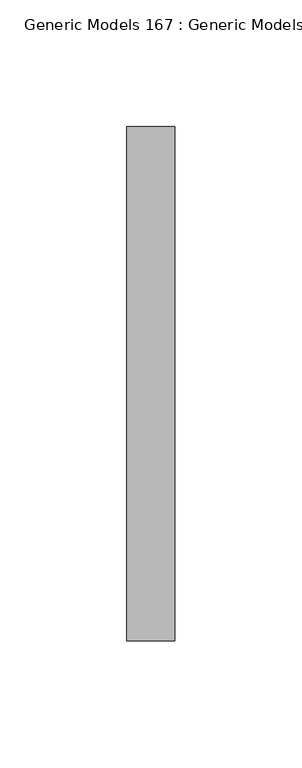
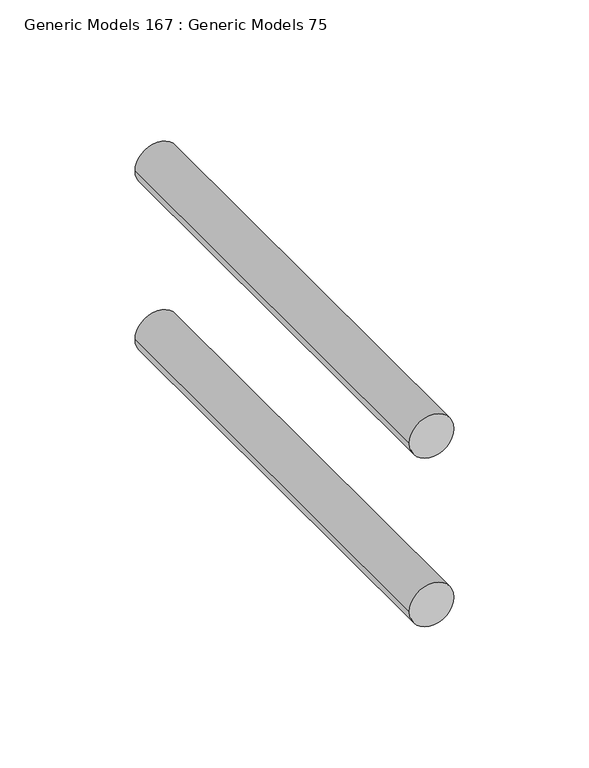
"""IFC4 building model written with IfcOpenShell, lengths in millimetres: proxy geometry, Generic Models 167 : Generic Models 75."""

from ifc_helpers import new_model, si_unit, point, frame, frame_2d, origin, place, context, project, spatial, circle_curve, trimmed, segment, composite_curve, outline, extrude, source, transform, mapped, element, save


def generic_models_167_generic_models_75_c1ef55c6(model_context):
    return source(origin(), model_context, "Body", "SweptSolid", [
        extrude(outline(composite_curve([segment(trimmed(circle_curve(frame_2d((271765.7125, 31975.4096032)), 9.525), [point((271765.7125, 31965.8846032))], [point((271765.7125, 31984.9346032))], False, "CARTESIAN"), True, "CONTINUOUS"), segment(trimmed(circle_curve(frame_2d((271765.7125, 31975.4096032)), 9.525), [point((271765.7125, 31984.9346032))], [point((271765.7125, 31965.8846032))], False, "CARTESIAN"), True, "CONTINUOUS")], self_intersect=False)), frame((0.0, 30672.7406612, 0.0), z_axis=(0.0, 1.0, 0.0), x_axis=(0.0, 0.0, 1.0)), (0.0, 0.0, 1.0), 203.2),
        extrude(outline(composite_curve([segment(trimmed(circle_curve(frame_2d((271841.9125, 31975.4096032)), 9.525), [point((271841.9125, 31965.8846032))], [point((271841.9125, 31984.9346032))], False, "CARTESIAN"), True, "CONTINUOUS"), segment(trimmed(circle_curve(frame_2d((271841.9125, 31975.4096032)), 9.525), [point((271841.9125, 31984.9346032))], [point((271841.9125, 31965.8846032))], False, "CARTESIAN"), True, "CONTINUOUS")], self_intersect=False)), frame((0.0, 30672.7406612, 0.0), z_axis=(0.0, 1.0, 0.0), x_axis=(0.0, 0.0, 1.0)), (0.0, 0.0, 1.0), 203.2),
    ])


if __name__ == "__main__":
    model = new_model("IFC4")
    model_context = context("Model", 3, world=origin())
    ifc_project = project(units=[si_unit("LENGTHUNIT", "METRE", prefix="MILLI")], contexts=[model_context])
    site = spatial("IfcSite", under=ifc_project)
    building = spatial("IfcBuilding", under=site)
    placement = place(None, origin())
    generic_models_167_generic_models_75_shape = generic_models_167_generic_models_75_c1ef55c6(model_context)
    element("IfcBuildingElementProxy", 1, Name="Generic Models 167 : Generic Models 75", ObjectType="Generic Models 167 : Generic Models 75", at=placement, inside=building, context=model_context, shape_type="MappedRepresentation", body=[
        mapped(generic_models_167_generic_models_75_shape, transform((0.0, 0.0, 0.0), x_axis=(1.0, 0.0, 0.0), y_axis=(0.0, 1.0, 0.0), z_axis=(0.0, 0.0, 1.0))),
    ])
    save(model, "model.ifc")
